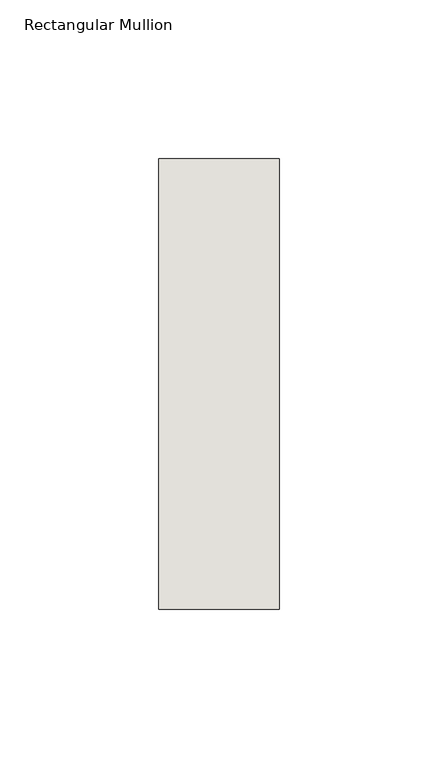
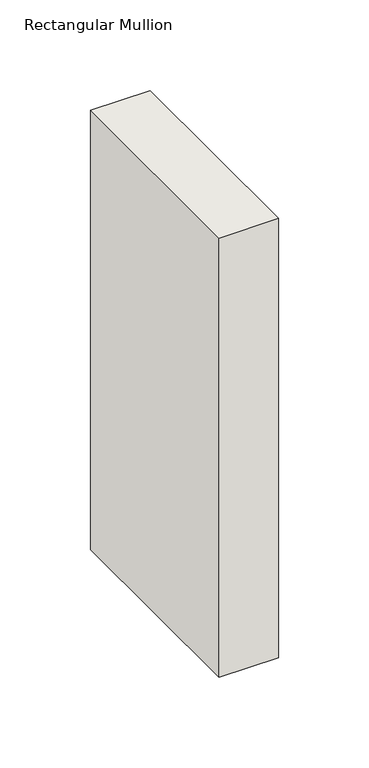
"""IFC4 building model written with IfcOpenShell, lengths in millimetres: wall geometry, Rectangular Mullion : NLRS_21_CWM_hsb-regel 38x142_gen_rsf."""

from ifc_helpers import new_model, si_unit, frame, origin, place, context, project, spatial, polyline, outline, extrude, source, transform, mapped, element, save


def rectangular_mullion_90e0555f(model_context):
    return source(origin(), model_context, "Body", "SweptSolid", [
        extrude(outline(polyline([(-38.0, -71.0), (-38.0, 71.0), (0.0, 71.0), (0.0, -71.0), (-38.0, -71.0)])), frame((0.0, 0.0, -296.0), z_axis=(0.0, 0.0, 1.0), x_axis=(1.0, 0.0, 0.0)), (0.0, 0.0, 1.0), 296.0),
    ])


if __name__ == "__main__":
    model = new_model("IFC4")
    model_context = context("Model", 3, world=origin())
    ifc_project = project(units=[si_unit("LENGTHUNIT", "METRE", prefix="MILLI")], contexts=[model_context])
    site = spatial("IfcSite", under=ifc_project)
    building = spatial("IfcBuilding", under=site)
    placement = place(None, origin())
    rectangular_mullion_shape = rectangular_mullion_90e0555f(model_context)
    element("IfcWall", 1, ObjectType="Rectangular Mullion : NLRS_21_CWM_hsb-regel 38x142_gen_rsf", at=placement, inside=building, context=model_context, shape_type="MappedRepresentation", body=[
        mapped(rectangular_mullion_shape, transform((0.0, 0.0, 0.0), x_axis=(1.0, 0.0, 0.0), y_axis=(0.0, 1.0, 0.0), z_axis=(0.0, 0.0, 1.0))),
    ])
    save(model, "model.ifc")

# Revit data of these elements
# Type "Rectangular Mullion : NLRS_21_CWM_hsb-regel 38x142_gen_rsf"
#   Type IfcGUID = "07M7mRoiH1CR8m_RSKIwpF"
#   Assembly Code = "21.10"
#   IfcExportAs = "IfcWall"
#   built-in parameter 1007322 = 0.465879 (stored number, unit not read)
#   built-in parameter 1007321 = 0.062336 (stored number, unit not read)
#   built-in parameter 1007320 = 0.062336 (stored number, unit not read)
# Element 1 (IfcWall, "Rectangular Mullion : NLRS_21_CWM_hsb-regel 38x142_gen_rsf")
#   Materials on its faces: "NLRS_i2_hout naaldhout vuren_gen_rsf"
# Materials
#   "NLRS_i2_hout naaldhout vuren_gen_rsf": class "I - Hout", colour RGB 234 199 147, transparency 0, Keynote = "i2", Manufacturer = "Revit Standards Foundation", URL = "www.revitstandards.org", Description = "hout vuren", Cost = 0
